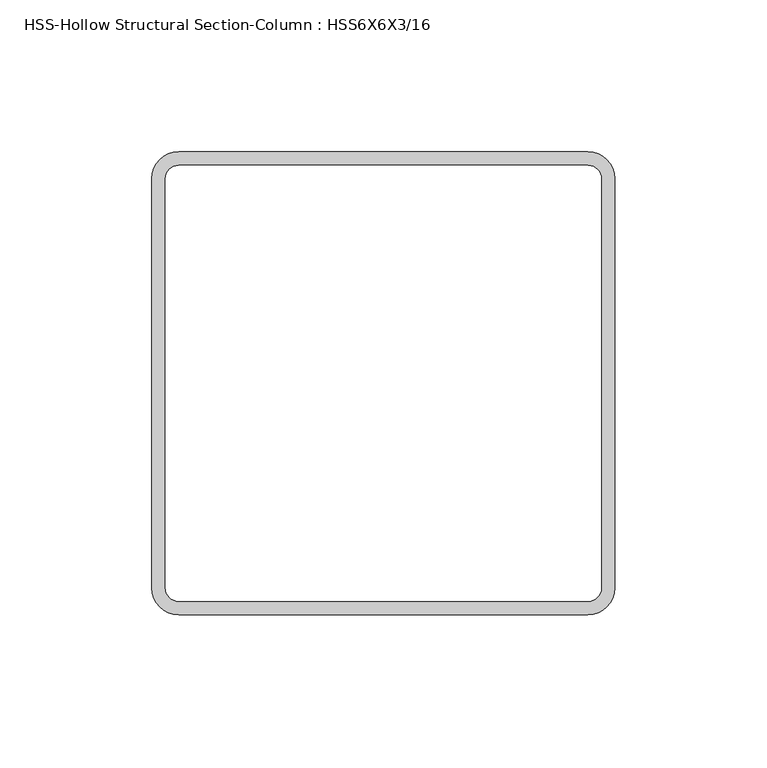
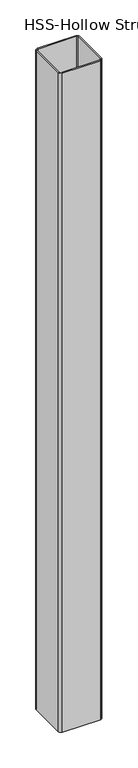
"""IFC4 building model written with IfcOpenShell, lengths in millimetres: column geometry, HSS-Hollow Structural Section-Column : HSS6X6X3/16."""

from ifc_helpers import new_model, si_unit, point, frame, frame_2d, origin, place, context, project, spatial, polyline, circle_curve, trimmed, segment, composite_curve, outline, extrude, source, transform, mapped, element, save


def hss_hollow_structural_section_column_hss6x6x3_16_e901b26d(model_context):
    return source(origin(), model_context, "Body", "SweptSolid", [
        extrude(outline(composite_curve([segment(trimmed(circle_curve(frame_2d((67.3608, 67.3608)), 8.8392), [point((67.3608, 76.2))], [point((76.2, 67.3608))], False, "CARTESIAN"), True, "CONTINUOUS"), segment(polyline([(76.2, 67.3608), (76.2, -67.3608)]), True, "CONTINUOUS"), segment(trimmed(circle_curve(frame_2d((67.3608, -67.3608)), 8.8392), [point((76.2, -67.3608))], [point((67.3608, -76.2))], False, "CARTESIAN"), True, "CONTINUOUS"), segment(polyline([(67.3608, -76.2), (-67.3608, -76.2)]), True, "CONTINUOUS"), segment(trimmed(circle_curve(frame_2d((-67.3608, -67.3608)), 8.8392), [point((-67.3608, -76.2))], [point((-76.2, -67.3608))], False, "CARTESIAN"), True, "CONTINUOUS"), segment(polyline([(-76.2, -67.3608), (-76.2, 67.3608)]), True, "CONTINUOUS"), segment(trimmed(circle_curve(frame_2d((-67.3608, 67.3608)), 8.8392), [point((-76.2, 67.3608))], [point((-67.3608, 76.2))], False, "CARTESIAN"), True, "CONTINUOUS"), segment(polyline([(-67.3608, 76.2), (67.3608, 76.2)]), True, "CONTINUOUS")], self_intersect=False), holes=[composite_curve([segment(polyline([(67.3608, 71.7804), (-67.3608, 71.7804)]), True, "CONTINUOUS"), segment(trimmed(circle_curve(frame_2d((-67.3608, 67.3608)), 4.4196), [point((-67.3608, 71.7804))], [point((-71.7804, 67.3608))], True, "CARTESIAN"), True, "CONTINUOUS"), segment(polyline([(-71.7804, 67.3608), (-71.7804, -67.3608)]), True, "CONTINUOUS"), segment(trimmed(circle_curve(frame_2d((-67.3608, -67.3608)), 4.4196), [point((-71.7804, -67.3608))], [point((-67.3608, -71.7804))], True, "CARTESIAN"), True, "CONTINUOUS"), segment(polyline([(-67.3608, -71.7804), (67.3608, -71.7804)]), True, "CONTINUOUS"), segment(trimmed(circle_curve(frame_2d((67.3608, -67.3608)), 4.4196), [point((67.3608, -71.7804))], [point((71.7804, -67.3608))], True, "CARTESIAN"), True, "CONTINUOUS"), segment(polyline([(71.7804, -67.3608), (71.7804, 67.3608)]), True, "CONTINUOUS"), segment(trimmed(circle_curve(frame_2d((67.3608, 67.3608)), 4.4196), [point((71.7804, 67.3608))], [point((67.3608, 71.7804))], True, "CARTESIAN"), True, "CONTINUOUS")], self_intersect=False)]), frame((0.0, 0.0, 3657.6), z_axis=(0.0, 0.0, 1.0), x_axis=(1.0, 0.0, 0.0)), (0.0, 0.0, 1.0), 2459.3898378),
    ])


if __name__ == "__main__":
    model = new_model("IFC4")
    model_context = context("Model", 3, world=origin())
    ifc_project = project(units=[si_unit("LENGTHUNIT", "METRE", prefix="MILLI")], contexts=[model_context])
    site = spatial("IfcSite", under=ifc_project)
    building = spatial("IfcBuilding", under=site)
    placement = place(None, origin())
    hss_hollow_structural_section_column_hss6x6x3_16_shape = hss_hollow_structural_section_column_hss6x6x3_16_e901b26d(model_context)
    element("IfcColumn", 1, ObjectType="HSS-Hollow Structural Section-Column : HSS6X6X3/16", at=placement, inside=building, context=model_context, shape_type="MappedRepresentation", body=[
        mapped(hss_hollow_structural_section_column_hss6x6x3_16_shape, transform((0.0, 0.0, 0.0), x_axis=(1.0, 0.0, 0.0), y_axis=(0.0, 1.0, 0.0), z_axis=(0.0, 0.0, 1.0))),
    ])
    save(model, "model.ifc")

# Revit data of these elements
# Type "HSS-Hollow Structural Section-Column : HSS6X6X3/16"
#   Assembly Code = "B10"
#   Shape = "Square"
#   W = 14.5
#   Ht = 0' - 6"
#   b = 0' - 6"
#   kr = 0' - 0.348"
#   t = 0' - 0.174"
#   A = 0.0276389 SF
#   Structural Material [instance default] = Steel ASTM A500, Grade B, Rectangular and Square
# Element 1 (IfcColumn, "HSS-Hollow Structural Section-Column : HSS6X6X3/16")
#   Structural Material = Steel
#   Materials on its faces: "Steel"
# Materials
#   "Steel ASTM A500, Grade B, Rectangular and Square": class "Metal", colour RGB 199 199 199, transparency 0, Description = "Carbon steel", Cost = 0
#   "Steel": class "Metal", colour RGB 118 118 114, transparency 0, Description = "Steel, mill finish", Cost = 0
